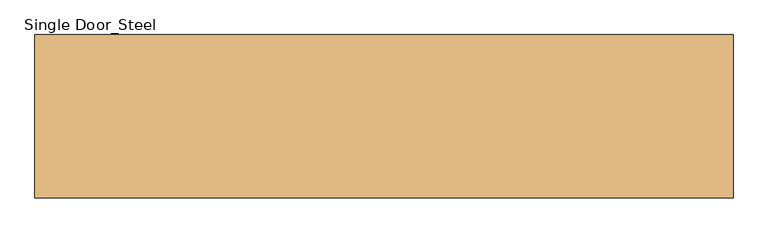
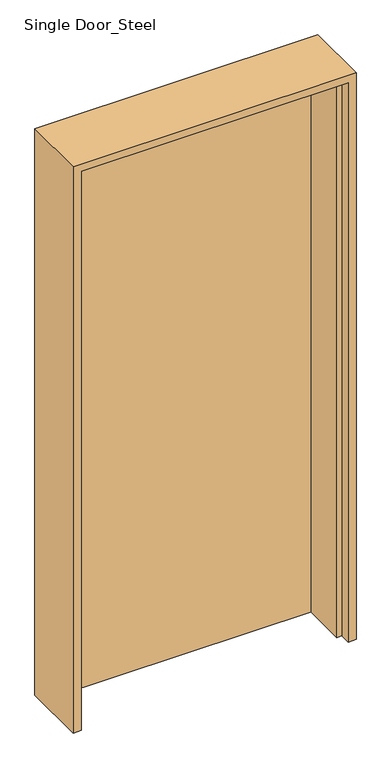
"""IFC4 building model written with IfcOpenShell, lengths in millimetres: door geometry, Single Door_Steel : H_DR_AR B12_Door_Single_W1100xH2280_FR 1.0H_FSD-1."""

from ifc_helpers import new_model, si_unit, origin, origin_with_axes, place, context, project, spatial, polyline, outline, extrude, faceted_brep, source, transform, mapped, element, save


def single_door_steel_ddb80ffe(model_context):
    return source(origin(), model_context, "Body", "SolidModel", [
        extrude(outline(polyline([(505.0, 125.0), (505.0, 85.0), (-505.0, 85.0), (-505.0, 125.0), (505.0, 125.0)])), origin_with_axes(), (0.0, 0.0, 1.0), 2235.0),
        faceted_brep([(505.0, 125.0, 0.0), (535.0, 125.0, 0.0), (535.0, -125.0, 0.0), (505.0, -125.0, 0.0), (505.0, -85.0, 0.0), (485.0, -85.0, 0.0), (485.0, 85.0, 0.0), (505.0, 85.0, 0.0), (-505.0, 125.0, 0.0), (-505.0, 85.0, 0.0), (-485.0, 85.0, 0.0), (-485.0, -85.0, 0.0), (-505.0, -85.0, 0.0), (-505.0, -125.0, 0.0), (-535.0, -125.0, 0.0), (-535.0, 125.0, 0.0), (505.0, 125.0, 2235.0), (-505.0, 125.0, 2235.0), (-535.0, 125.0, 2265.0), (535.0, 125.0, 2265.0), (535.0, -125.0, 2265.0), (-535.0, -125.0, 2265.0), (-505.0, -125.0, 2235.0), (505.0, -125.0, 2235.0), (505.0, -85.0, 2235.0), (-505.0, -85.0, 2235.0), (-485.0, -85.0, 2215.0), (485.0, -85.0, 2215.0), (485.0, 85.0, 2215.0), (-485.0, 85.0, 2215.0), (-505.0, 85.0, 2235.0), (505.0, 85.0, 2235.0)], [[[0, 1, 2, 3, 4, 5, 6, 7]], [[8, 9, 10, 11, 12, 13, 14, 15]], [[1, 0, 16, 17, 8, 15, 18, 19]], [[2, 1, 19, 20]], [[3, 2, 20, 21, 14, 13, 22, 23]], [[4, 3, 23, 24]], [[5, 4, 24, 25, 12, 11, 26, 27]], [[6, 5, 27, 28]], [[7, 6, 28, 29, 10, 9, 30, 31]], [[0, 7, 31, 16]], [[17, 30, 9, 8]], [[21, 18, 15, 14]], [[25, 22, 13, 12]], [[29, 26, 11, 10]], [[20, 19, 18, 21]], [[24, 23, 22, 25]], [[28, 27, 26, 29]], [[16, 31, 30, 17]]]),
    ])


if __name__ == "__main__":
    model = new_model("IFC4")
    model_context = context("Model", 3, world=origin())
    ifc_project = project(units=[si_unit("LENGTHUNIT", "METRE", prefix="MILLI")], contexts=[model_context])
    site = spatial("IfcSite", under=ifc_project)
    building = spatial("IfcBuilding", under=site)
    placement = place(None, origin())
    single_door_steel_shape = single_door_steel_ddb80ffe(model_context)
    element("IfcDoor", 1, ObjectType="Single Door_Steel : H_DR_AR B12_Door_Single_W1100xH2280_FR 1.0H_FSD-1", at=placement, inside=building, context=model_context, shape_type="MappedRepresentation", body=[
        mapped(single_door_steel_shape, transform((0.0, 0.0, 0.0), x_axis=(1.0, 0.0, 0.0), y_axis=(0.0, 1.0, 0.0), z_axis=(0.0, 0.0, 1.0))),
    ])
    save(model, "model.ifc")

# Revit data of these elements
# Type "Single Door_Steel : H_DR_AR B12_Door_Single_W1100xH2280_FR 1.0H_FSD-1"
#   Type Mark = "441"
#   Analytic Construction = "<None>"
#   프레임 투영 외부. = 25 mm
#   프레임 투영 내부. = 25 mm
#   프레임 폭 = 75 mm
#   Height = 2280 mm
#   Width = 1100 mm
#   Define Thermal Properties by = 1
#   문 패널 = none
#   문 프레임 = none
#   Function = (empty or 0)
#   Wall Closure = (empty or 0)
